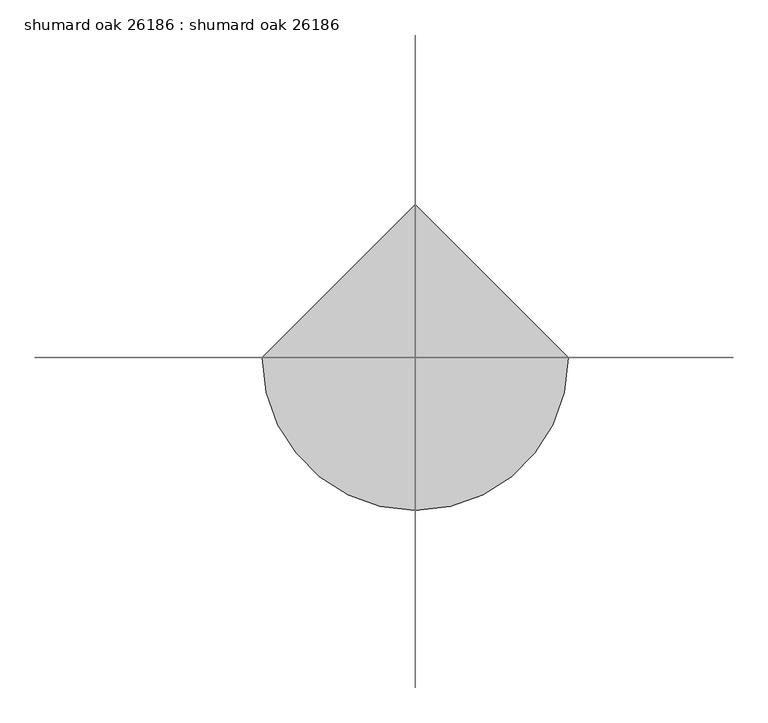
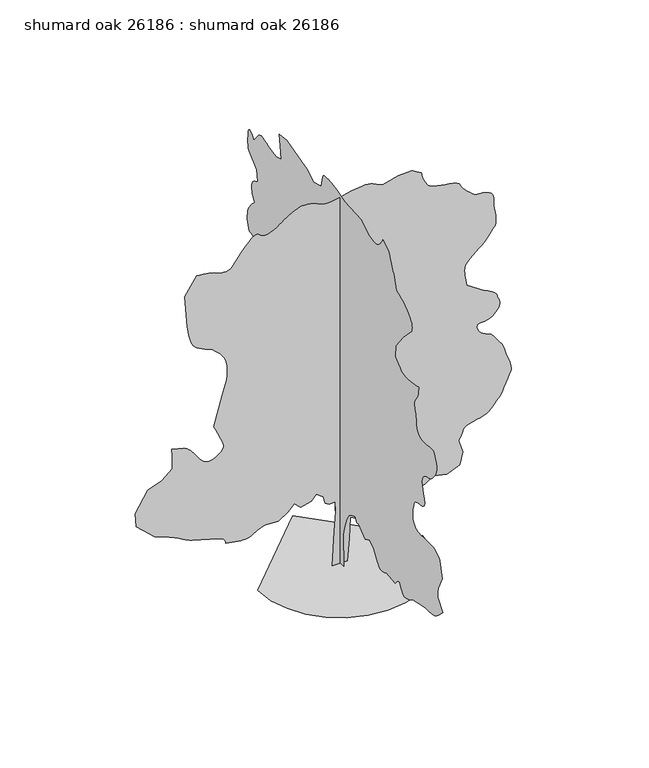
"""IFC4 building model written with IfcOpenShell, lengths in millimetres: proxy geometry, shumard oak 26186 : shumard oak 26186."""

from ifc_helpers import new_model, si_unit, origin, place, context, project, spatial, triangles, source, transform, mapped, element, save


def shumard_oak_26186_shumard_oak_26186_cf07c7db(model_context):
    return source(origin(), model_context, "Body", "Tessellation", [
        triangles([(-0.0016958, 164.6246354, 0.0086022), (-0.0016958, -151.6104316, 0.0086022), (-0.0016958, -124.1113561, 783.7227293), (-0.0016958, -179.1089983, 1017.4612965), (-0.0016958, -261.6049622, 1237.4509209), (-0.0016958, -357.8507226, 1388.6927067), (-0.0016958, -467.8454985, 1457.4403999), (-0.0016958, -605.3383779, 1512.436607), (-0.0016958, -660.3370193, 1388.6927067), (-0.0016958, -756.5828161, 1416.1908829), (-0.0016958, -866.5775557, 1306.195998), (-0.0016958, -1017.8194868, 1209.9502739), (-0.0016958, -1196.5619196, 1292.4469826), (-0.0016958, -1361.5527935, 1182.452243), (-0.0016958, -1471.5476784, 989.9607222), (-0.0016958, -1498.1643677, 951.9597713), (-0.0016958, -1525.3829098, 915.7621988), (-0.0016958, -1553.8031227, 883.1739264), (-0.0016958, -1584.0290394, 855.9959341), (-0.0016958, -1616.658007, 836.0340712), (-0.0016958, -1652.2942039, 825.0891724), (-0.0016958, -1691.5371574, 824.9697756), (-0.0016958, -1729.1774471, 831.662681), (-0.0016958, -1760.3255459, 839.8008471), (-0.0016958, -1786.0582775, 849.1404659), (-0.0016958, -1807.4654011, 859.4426714), (-0.0016958, -1825.6238857, 870.4663445), (-0.0016958, -1841.6182583, 881.9725462), (-0.0016958, -1856.5307201, 893.7149254), (-0.0016958, -2214.0131149, 852.4678791), (-0.0016958, -2249.2480282, 893.1561659), (-0.0016958, -2283.7616192, 930.4738735), (-0.0016958, -2316.8324203, 961.0605967), (-0.0016958, -2347.7391094, 981.54314), (-0.0016958, -2375.7578934, 988.5586275), (-0.0016958, -2400.1697754, 978.7389507), (-0.0016958, -2420.2535786, 948.7136032), (-0.0016958, -2440.416156, 905.5412384), (-0.0016958, -2465.389341, 860.9260838), (-0.0016958, -2494.9323051, 818.4750412), (-0.0016958, -2528.8058189, 781.7974108), (-0.0016958, -2566.7735596, 754.4999491), (-0.0016958, -2608.5820541, 740.1896307), (-0.0016958, -2653.9973053, 742.4730669), (-0.0016958, -2699.5395836, 755.8614212), (-0.0016958, -2742.1861084, 772.1352098), (-0.0016958, -2782.4196991, 790.8169184), (-0.0016958, -2820.7484642, 811.421402), (-0.0016958, -2857.6293526, 833.4686754), (-0.0016958, -2893.5448929, 856.475992), (-0.0016958, -2928.9779045, 879.96591), (-0.0016958, -3423.9482735, 976.2117067), (-0.0016958, -3485.6956673, 976.3335743), (-0.0016958, -3546.579451, 977.174366), (-0.0016958, -3605.7868835, 979.4603456), (-0.0016958, -3662.4543549, 983.9078939), (-0.0016958, -3715.7688332, 991.2459635), (-0.0016958, -3764.8925789, 1002.1882462), (-0.0016958, -3808.9361115, 1017.4612965), (-0.0016958, -3851.3797417, 1039.546649), (-0.0016958, -3896.0075409, 1069.5719965), (-0.0016958, -3942.4134293, 1106.2115479), (-0.0016958, -3990.2924835, 1148.1393665), (-0.0016958, -4039.2383331, 1194.0371464), (-0.0016958, -4088.8951859, 1242.5817123), (-0.0016958, -4138.9334106, 1292.4469826), (-0.0016958, -3946.4265564, 1512.436607), (-0.0016958, -3940.7114983, 1553.6455742), (-0.0016958, -3935.9362083, 1594.6132771), (-0.0016958, -3933.0916145, 1635.0983059), (-0.0016958, -3933.1169037, 1674.8646286), (-0.0016958, -3937.0032944, 1713.6657486), (-0.0016958, -3945.7152626, 1751.2679592), (-0.0016958, -3960.1934486, 1787.4247639), (-0.0016958, -4111.425206, 2103.6601124), (-0.0016958, -4015.1842781, 2488.640538), (-0.0016958, -4007.6405525, 2499.2628548), (-0.0016958, -3985.1869812, 2526.4815422), (-0.0016958, -3948.0776184, 2563.3191193), (-0.0016958, -3896.5156494, 2602.8164177), (-0.0016958, -3830.780127, 2637.9697952), (-0.0016958, -3751.1003975, 2661.820665), (-0.0016958, -3657.7046448, 2667.3831161), (-0.0016958, -3553.6406479, 2663.0650658), (-0.0016958, -3446.4524231, 2661.3634254), (-0.0016958, -3343.1000107, 2661.617189), (-0.0016958, -3250.5928665, 2663.0650658), (-0.0016958, -3175.8660324, 2664.970182), (-0.0016958, -3125.9298363, 2666.6718224), (-0.0016958, -3107.7178665, 2667.3831161), (-0.0016958, -3097.049913, 2674.6474983), (-0.0016958, -3069.5669975, 2695.1200859), (-0.0016958, -3031.9495262, 2726.9207611), (-0.0016958, -2990.9793526, 2768.0688309), (-0.0016958, -2953.3874611, 2816.7097572), (-0.0016958, -2925.9045456, 2870.8625565), (-0.0016958, -2915.2365921, 2928.622403), (-0.0016958, -2917.2431557, 2986.3310898), (-0.0016958, -2922.8564758, 3041.9064766), (-0.0016958, -2931.4672874, 3095.6529053), (-0.0016958, -2942.4907425, 3147.977037), (-0.0016958, -2955.3178665, 3199.2087936), (-0.0016958, -2969.3385223, 3249.7039673), (-0.0016958, -2983.9690247, 3299.8436394), (-0.0016958, -2996.0086967, 3314.52472), (-0.0016958, -3009.4706657, 3328.8250099), (-0.0016958, -3025.8280975, 3342.414006), (-0.0016958, -3046.5038704, 3354.9362068), (-0.0016958, -3072.9705688, 3365.9852417), (-0.0016958, -3106.6510712, 3375.2561874), (-0.0016958, -3148.9673836, 3382.3429642), (-0.0016958, -3200.1485619, 3386.6863037), (-0.0016958, -3255.4443146, 3391.740937), (-0.0016958, -3308.7843727, 3403.2725006), (-0.0016958, -3354.1996239, 3427.0722107), (-0.0016958, -3385.6703773, 3468.9315742), (-0.0016958, -3397.1766518, 3534.5906479), (-0.0016958, -3382.6984657, 3629.8406479), (-0.0016958, -3353.0819595, 3737.5114014), (-0.0016958, -3325.8786781, 3836.2667107), (-0.0016958, -3305.152327, 3925.6746254), (-0.0016958, -3294.9921913, 4005.2023293), (-0.0016958, -3299.5387161, 4074.3920013), (-0.0016958, -3322.8306084, 4132.761113), (-0.0016958, -3368.9571533, 4179.8018463), (-0.0016958, -3425.5228867, 4212.7710548), (-0.0016958, -3477.9993347, 4232.964299), (-0.0016958, -3527.3262657, 4246.1975029), (-0.0016958, -3574.5193153, 4258.2118858), (-0.0016958, -3620.493544, 4274.8233719), (-0.0016958, -3666.2390076, 4301.7473099), (-0.0016958, -3712.6954742, 4344.8004959), (-0.0016958, -3760.0411308, 4399.562851), (-0.0016958, -3805.2023277, 4457.9322533), (-0.0016958, -3844.3694138, 4520.1368866), (-0.0016958, -3873.6809967, 4586.4308052), (-0.0016958, -3889.2765564, 4657.068354), (-0.0016958, -3887.295282, 4732.2777168), (-0.0016958, -3863.9272316, 4812.2879494), (-0.0016958, -3835.7077332, 4887.9545517), (-0.0016958, -3816.632444, 4949.7019455), (-0.0016958, -3799.0047409, 4996.9967331), (-0.0016958, -3775.1032928, 5029.3819656), (-0.0016958, -3737.2573471, 5046.3745331), (-0.0016958, -3677.7705711, 5047.4919067), (-0.0016958, -3588.9466324, 5032.2771378), (-0.0016958, -3483.5620766, 5015.437468), (-0.0016958, -3382.266806, 5012.0591858), (-0.0016958, -3289.150106, 5022.1684525), (-0.0016958, -3208.3018433, 5045.7396881), (-0.0016958, -3143.7860138, 5082.7728928), (-0.0016958, -3099.7421906, 5133.2930649), (-0.0016958, -3080.2096619, 5197.2507889), (-0.0016958, -3073.5295464, 5265.5768509), (-0.0016958, -3065.4015541, 5329.5339935), (-0.0016958, -3056.0541595, 5389.9099594), (-0.0016958, -3045.7417076, 5447.3901718), (-0.0016958, -3034.7182526, 5502.7112137), (-0.0016958, -3023.2119781, 5556.5846695), (-0.0016958, -3011.4772293, 5609.7471222), (-0.0016958, -3000.047113, 5648.0755966), (-0.0016958, -2990.8014565, 5686.505809), (-0.0016958, -2985.8485611, 5725.1900757), (-0.0016958, -2987.423465, 5764.2295532), (-0.0016958, -2997.6341789, 5803.7521408), (-0.0016958, -3018.6907425, 5843.8839935), (-0.0016958, -3052.7267464, 5884.7274307), (-0.0016958, -3089.125106, 5934.8418137), (-0.0016958, -3116.6080215, 5997.6815826), (-0.0016958, -3136.4198936, 6065.8297485), (-0.0016958, -3149.7295464, 6131.8187439), (-0.0016958, -3157.7558006, 6188.1815826), (-0.0016958, -3161.6674805, 6227.450116), (-0.0016958, -3162.7089867, 6242.2073547), (-0.0016958, -3142.4395844, 6237.6861191), (-0.0016958, -3088.0074417, 6226.1798447), (-0.0016958, -3009.0387154, 6210.8383392), (-0.0016958, -2915.160434, 6194.7602509), (-0.0016958, -2815.9731743, 6181.0948059), (-0.0016958, -2721.1295448, 6172.9418152), (-0.0016958, -2640.2304131, 6173.4749222), (-0.0016958, -2571.9299309, 6185.3619873), (-0.0016958, -2507.9599983, 6208.094902), (-0.0016958, -2447.5915901, 6239.8452896), (-0.0016958, -2390.1089069, 6278.808609), (-0.0016958, -2334.7901905, 6323.1826447), (-0.0016958, -2280.9167347, 6371.1634369), (-0.0016958, -2227.7621304, 6420.9476074), (-0.0016958, -2241.5111458, 6709.6945175), (-0.0016958, -2543.9897758, 7094.6826462), (-0.0016958, -2887.7283875, 7452.1625702), (-0.0016958, -2893.1132332, 7496.4860275), (-0.0016958, -2895.3482712, 7541.6722229), (-0.0016958, -2891.335144, 7588.5356415), (-0.0016958, -2877.9493332, 7637.9128601), (-0.0016958, -2852.0666107, 7690.6689423), (-0.0016958, -2810.5377502, 7747.6160477), (-0.0016958, -2750.2379425, 7809.6424942), (-0.0016958, -2679.5242355, 7869.2562973), (-0.0016958, -2608.8108192, 7919.4724182), (-0.0016958, -2538.10467, 7961.8901779), (-0.0016958, -2467.3935791, 7998.0344833), (-0.0016958, -2396.6824883, 8029.5052368), (-0.0016958, -2325.9712521, 8057.8517624), (-0.0016958, -2255.2601612, 8084.6233841), (-0.0016958, -2234.6175259, 8155.1336151), (-0.0016958, -2213.8530956, 8224.4503143), (-0.0016958, -2192.8472557, 8291.3537888), (-0.0016958, -2171.4808273, 8354.651088), (-0.0016958, -2149.6341957, 8413.1219376), (-0.0016958, -2127.1881821, 8465.5983856), (-0.0016958, -2104.0183754, 8510.8607391), (-0.0016958, -2078.3235775, 8560.2129593), (-0.0016958, -2049.9822842, 8621.0970337), (-0.0016958, -2021.4021973, 8686.5529221), (-0.0016958, -1994.9862225, 8749.5955856), (-0.0016958, -1973.1395908, 8803.2917267), (-0.0016958, -1958.2679695, 8840.6039841), (-0.0016958, -1952.7738281, 8854.5996414), (-0.0016958, -1719.0353336, 8992.089505), (-0.0016958, -1707.0516174, 8968.3915329), (-0.0016958, -1693.863905, 8943.9819763), (-0.0016958, -1678.2681999, 8918.1248337), (-0.0016958, -1659.0683544, 8890.1085205), (-0.0016958, -1635.057756, 8859.1970352), (-0.0016958, -1605.0324085, 8824.678212), (-0.0016958, -1567.7934025, 8785.841629), (-0.0016958, -1522.9369835, 8752.2122864), (-0.0016958, -1471.5882282, 8732.2983856), (-0.0016958, -1414.8268673, 8723.7896027), (-0.0016958, -1353.7372822, 8724.4244476), (-0.0016958, -1289.3990582, 8731.9175949), (-0.0016958, -1222.896722, 8743.9825562), (-0.0016958, -1155.3123299, 8758.3334244), (-0.0016958, -852.8259968, 8964.5813004), (-0.0016958, -192.8582863, 9005.8311081), (-0.0016958, -107.5965211, 9029.2756073), (-0.0016958, -23.416737, 9052.008522), (-0.0016958, 58.5983536, 9073.2938507), (-0.0016958, 137.366361, 9092.4200089), (-0.0016958, 211.8051857, 9108.6504135), (-0.0016958, 280.8327856, 9121.2740616), (-0.0016958, 343.3650879, 9129.57995), (-0.0016958, 405.0185557, 9135.9045639), (-0.0016958, 469.5549508, 9141.5181747), (-0.0016958, 533.1311937, 9144.0075577), (-0.0016958, 591.8966838, 9140.9594879), (-0.0016958, 642.0033274, 9129.9863205), (-0.0016958, 679.6029219, 9108.6504135), (-0.0016958, 700.8500261, 9074.5891205), (-0.0016958, 769.5952486, 8799.5832321), (-0.0016958, 1072.081509, 8717.1091965), (-0.0016958, 1347.0698112, 8882.0822662), (-0.0016958, 1690.8031906, 8964.5813004), (-0.0016958, 2144.5313095, 9102.0717453), (-0.0016958, 2447.0174973, 9060.8225189), (-0.0016958, 2419.5169956, 8799.5832321), (-0.0016958, 2364.5209339, 8497.1197174), (-0.0016958, 2584.5030006, 8428.361705), (-0.0016958, 2804.4924797, 8469.6115128), (-0.0016958, 2889.5570549, 8501.5647949), (-0.0016958, 2972.3357231, 8530.7490601), (-0.0016958, 3050.5425774, 8554.3964539), (-0.0016958, 3121.8911293, 8569.7385406), (-0.0016958, 3184.1210518, 8574.0307205), (-0.0016958, 3234.8958595, 8564.480722), (-0.0016958, 3271.9799332, 8538.3439453), (-0.0016958, 3478.2280998, 8290.8712601), (-0.0016958, 3525.090937, 8345.6591949), (-0.0016958, 3570.2521339, 8393.3603531), (-0.0016958, 3612.0606285, 8426.8885391), (-0.0016958, 3648.8144897, 8439.1058167), (-0.0016958, 3678.8373665, 8422.9515701), (-0.0016958, 3700.4526169, 8371.313443), (-0.0016958, 3711.9588913, 8277.1046585), (-0.0016958, 3715.4389114, 8172.4819748), (-0.0016958, 3714.6005905, 8091.684581), (-0.0016958, 3710.155513, 8030.6987686), (-0.0016958, 3702.8149727, 7985.6137299), (-0.0016958, 3693.3152618, 7952.4163376), (-0.0016958, 3682.3679649, 7927.1684601), (-0.0016958, 3670.7093742, 7905.8831314), (-0.0016958, 3354.4789673, 7644.6438446), (-0.0016958, 3326.9707626, 7355.921933), (-0.0016958, 3370.9384277, 7337.989888), (-0.0016958, 3413.6102417, 7318.6346741), (-0.0016958, 3453.615358, 7296.384288), (-0.0016958, 3489.6326363, 7269.8161423), (-0.0016958, 3520.3920959, 7237.4564896), (-0.0016958, 3544.5220184, 7197.8833237), (-0.0016958, 3560.7018448, 7149.674057), (-0.0016958, 3566.8994316, 7096.6389221), (-0.0016958, 3562.9624626, 7043.6032059), (-0.0016958, 3550.618158, 6990.568071), (-0.0016958, 3531.5425781, 6937.5329361), (-0.0016958, 3507.4126556, 6884.4978012), (-0.0016958, 3479.904451, 6831.4626663), (-0.0016958, 3450.7198952, 6778.4269501), (-0.0016958, 3494.7381386, 6734.2313919), (-0.0016958, 3537.6640068, 6689.8829361), (-0.0016958, 3578.4309952, 6645.3060059), (-0.0016958, 3615.9470192, 6600.3732834), (-0.0016958, 3649.1447021, 6554.9580322), (-0.0016958, 3676.9322502, 6508.9329346), (-0.0016958, 3698.2175789, 6462.1968338), (-0.0016958, 3713.4829262, 6416.6548462), (-0.0016958, 3724.4305138, 6374.0080307), (-0.0016958, 3731.7710541, 6333.77444), (-0.0016958, 3736.2161316, 6295.4459656), (-0.0016958, 3738.5020386, 6258.5650772), (-0.0016958, 3739.3400688, 6222.6492462), (-0.0016958, 3739.4670959, 6187.2165253), (-0.0016958, 3656.9680618, 5953.4854431), (-0.0016958, 3618.6901657, 5947.3387253), (-0.0016958, 3580.5140076, 5939.7694199), (-0.0016958, 3542.591613, 5929.304361), (-0.0016958, 3505.0250107, 5914.5215424), (-0.0016958, 3467.9665169, 5893.9477982), (-0.0016958, 3431.4664192, 5866.1599594), (-0.0016958, 3395.728775, 5829.7366013), (-0.0016958, 3363.165937, 5786.4799393), (-0.0016958, 3335.6830215, 5739.6171021), (-0.0016958, 3312.3911293, 5689.7567734), (-0.0016958, 3292.4522301, 5637.4838013), (-0.0016958, 3275.0532921, 5583.4068695), (-0.0016958, 3259.3559944, 5528.1364059), (-0.0016958, 3244.4717285, 5472.2566772), (-0.0016958, 3212.2896812, 5428.0349579), (-0.0016958, 3181.4287743, 5383.7120819), (-0.0016958, 3153.2092758, 5339.1351517), (-0.0016958, 3128.9523262, 5294.1768494), (-0.0016958, 3110.0037735, 5248.7615982), (-0.0016958, 3097.6341797, 5202.7620804), (-0.0016958, 3093.2399712, 5156.026561), (-0.0016958, 3106.9812836, 4784.7797447), (-0.0016958, 3139.1630402, 4781.5284897), (-0.0016958, 3170.049527, 4776.4738564), (-0.0016958, 3198.2690254, 4767.8377556), (-0.0016958, 3222.5006859, 4753.7662308), (-0.0016958, 3241.4745277, 4732.4809021), (-0.0016958, 3253.8188324, 4702.1533928), (-0.0016958, 3258.2383301, 4661.0306122), (-0.0016958, 3257.0192184, 4613.5073502), (-0.0016958, 3253.6665161, 4565.2219254), (-0.0016958, 3248.4848557, 4516.377523), (-0.0016958, 3241.8808983, 4467.0253029), (-0.0016958, 3234.1845657, 4417.3175812), (-0.0016958, 3225.7516502, 4367.3810944), (-0.0016958, 3216.988813, 4317.2922913), (-0.0016958, 3203.2219208, 4042.311692), (-0.0016958, 3464.4612076, 4056.0785843), (-0.0016958, 3753.208699, 4111.0694138), (-0.0016958, 3814.6511696, 4090.2669044), (-0.0016958, 3873.5792587, 4068.37202), (-0.0016958, 3927.4527145, 4044.3182556), (-0.0016958, 3973.7568649, 4017.0132362), (-0.0016958, 4009.9520393, 3985.3901665), (-0.0016958, 4033.523275, 3948.3569618), (-0.0016958, 4041.9306107, 3904.8212471), (-0.0016958, 4039.5429657, 3849.6778107), (-0.0016958, 4032.8119812, 3780.081768), (-0.0016958, 4022.448951, 3698.4716331), (-0.0016958, 4009.2407455, 3607.2347603), (-0.0016958, 3993.8483711, 3508.7840836), (-0.0016958, 3977.00812, 3405.5078293), (-0.0016958, 3959.4568657, 3299.8436394), (-0.0016958, 3835.7077332, 2969.87192), (-0.0016958, 3768.1185448, 2931.9498161), (-0.0016958, 3701.6211502, 2896.3136192), (-0.0016958, 3637.2829262, 2865.2492363), (-0.0016958, 3576.1959572, 2841.0431557), (-0.0016958, 3519.4267479, 2825.9554138), (-0.0016958, 3468.0679642, 2822.3233681), (-0.0016958, 3423.2113998, 2832.3817657), (-0.0016958, 3038.248851, 2997.3548355), (-0.0016958, 2653.2607224, 2873.6312828), (-0.0016958, 2378.2699493, 2681.1244286), (-0.0016958, 2103.2842632, 2268.651059), (-0.0016958, 2076.6675739, 2227.6428062), (-0.0016958, 2049.4488865, 2188.0796688), (-0.0016958, 2021.0263481, 2151.4021111), (-0.0016958, 1990.8027569, 2119.0526321), (-0.0016958, 1958.1739346, 2092.4764927), (-0.0016958, 1922.5377377, 2073.1141571), (-0.0016958, 1883.2946388, 2062.4105953), (-0.0016958, 1844.1303143, 2058.8443886), (-0.0016958, 1807.3715115, 2059.123732), (-0.0016958, 1770.371299, 2062.0498615), (-0.0016958, 1730.4881229, 2066.4186356), (-0.0016958, 1685.070401, 2071.0288193), (-0.0016958, 1631.4762886, 2074.6762711), (-0.0016958, 1567.0592903, 2076.1596107), (-0.0016958, 1497.9510086, 2070.950045), (-0.0016958, 1431.730632, 2056.3577671), (-0.0016958, 1367.9130157, 2033.9498325), (-0.0016958, 1306.020718, 2005.2883553), (-0.0016958, 1245.5712101, 1971.9382107), (-0.0016958, 1186.0844341, 1935.4612221), (-0.0016958, 1127.0801868, 1897.4196487), (-0.0016958, 1044.5834782, 1663.6810089), (-0.0016958, 810.8448383, 1402.4418674), (-0.0016958, 778.5741337, 1367.4862976), (-0.0016958, 741.256426, 1333.2546661), (-0.0016958, 699.7273476, 1299.622562), (-0.0016958, 654.8303061, 1266.4729866), (-0.0016958, 607.408455, 1233.6815289), (-0.0016958, 558.3051295, 1201.1339516), (-0.0016958, 508.3585416, 1168.7032276), (-0.0016958, 425.8618329, 1457.4403999), (-0.0016958, 288.3689717, 1649.9293774), (-0.0016958, 233.3715837, 1526.1856224), (-0.0016958, 192.1232112, 1333.696645), (-0.0016958, 178.3741776, 989.9607222), (-0.0016958, 150.8753565, 508.7344634), (170.3625119, 0.000436, 0.0217742), (-187.1199193, 0.000436, 0.0217742), (-132.1230309, 0.000387, 824.9824928), (-104.6242098, 0.0003581, 1306.2087879), (-118.3734886, 0.0003434, 1553.698914), (-255.8671038, 0.0003442, 1539.9498985), (-352.1128461, 0.000341, 1594.9459602), (-393.359965, 0.0003302, 1773.6885384), (-558.3534187, 0.0003237, 1883.6832779), (-668.3482309, 0.000331, 1759.9395229), (-915.8358135, 0.0003352, 1691.1918297), (-1067.0802881, 0.0003271, 1828.6846001), (-1218.3221466, 0.000336, 1677.4428143), (-1438.311771, 0.0003442, 1539.9498985), (-1768.2961349, 0.0003434, 1553.698914), (-1933.2869362, 0.0003476, 1484.9512207), (-1968.7250347, 0.0003491, 1458.6138748), (-2004.6407204, 0.0003507, 1433.3612011), (-2041.5189926, 0.000352, 1410.2726395), (-2079.8425255, 0.0003531, 1390.4301006), (-2120.0889061, 0.0003541, 1374.915786), (-2162.738047, 0.0003547, 1364.8142223), (-2208.2752384, 0.0003549, 1361.2074657), (-2259.0244663, 0.0003549, 1362.8101295), (-2316.2658852, 0.0003547, 1367.3008438), (-2378.9175842, 0.0003541, 1374.1944637), (-2445.902449, 0.0003536, 1383.0132568), (-2516.1310112, 0.0003531, 1393.2749851), (-2588.5161278, 0.0003523, 1404.4991547), (-2661.9982704, 0.0003518, 1416.2061436), (-2665.4018417, 0.0003499, 1445.5887978), (-2671.5741394, 0.0003481, 1474.4889233), (-2683.2835991, 0.0003465, 1502.428933), (-2703.2986565, 0.0003449, 1528.9262981), (-2734.3630394, 0.0003434, 1553.4981995), (-2779.2448929, 0.0003421, 1575.6648697), (-2840.7382324, 0.000341, 1594.9459602), (-3445.7158401, 0.0003302, 1773.6885384), (-3495.0936401, 0.0003295, 1789.3602562), (-3547.8494316, 0.0003281, 1811.5293972), (-3602.2815742, 0.0003266, 1838.265556), (-3656.7140076, 0.0003247, 1867.6482101), (-3709.469799, 0.0003229, 1897.7523319), (-3758.8728882, 0.0003213, 1926.6550735), (-3803.1957642, 0.0003197, 1952.4285004), (-3850.8716331, 0.0003182, 1977.2011162), (-3910.0790657, 0.0003166, 2004.1403149), (-3978.8876564, 0.0003148, 2032.8804211), (-4055.4181595, 0.0003132, 2063.0657879), (-4137.7140083, 0.0003113, 2094.3332108), (-4223.8456696, 0.0003092, 2126.3194851), (-4311.9327347, 0.0003074, 2158.668964), (-4738.1450912, 0.0002835, 2557.4011665), (-4765.6532959, 0.0002638, 2887.3725952), (-4476.9060951, 0.000236, 3354.8600487), (-4146.9343758, 0.0002287, 3478.6088905), (-3899.4364014, 0.0002163, 3684.8570572), (-3899.4364014, 0.0001977, 4001.0874641), (-3913.2032936, 0.0001877, 4166.0858231), (-3624.4558022, 0.0001919, 4097.3281013), (-3591.9438332, 0.0001932, 4076.3729851), (-3558.8475975, 0.0001945, 4053.3607269), (-3524.5322502, 0.0001961, 4026.2588928), (-3488.4135246, 0.0001979, 3993.03563), (-3449.8815742, 0.0002006, 3951.6082169), (-3408.3524231, 0.0002037, 3899.9953789), (-3363.216806, 0.0002074, 3836.0888145), (-3317.4713425, 0.0002113, 3768.956575), (-3273.4275192, 0.000215, 3709.7491425), (-3229.3839867, 0.0002179, 3659.6856285), (-3183.6385231, 0.0002203, 3619.9601463), (-3134.5403572, 0.0002221, 3591.765937), (-3080.387558, 0.0002229, 3576.3482735), (-3019.4781944, 0.0002229, 3574.8495277), (-2952.9046417, 0.0002221, 3590.0895859), (-2885.848851, 0.0002203, 3620.9507835), (-2822.8567657, 0.0002176, 3662.8860146), (-2768.5513596, 0.0002147, 3711.2984665), (-2727.4541588, 0.0002119, 3761.6413239), (-2704.1622665, 0.000209, 3809.3427727), (-2703.2480782, 0.0002066, 3849.8304176), (-2719.4531937, 0.000204, 3893.6198959), (-2743.5831161, 0.0002006, 3952.5479851), (-2774.3172867, 0.0001961, 4024.0997223), (-2810.3598541, 0.0001914, 4105.735437), (-2850.3649704, 0.0001861, 4194.9657463), (-2893.0114952, 0.0001803, 4289.2506889), (-2936.9788696, 0.0001746, 4386.0755928), (-2744.4975952, 0.0001328, 5087.2685486), (-2718.1576332, 0.0001281, 5166.6433548), (-2692.9100464, 0.0001234, 5244.9263672), (-2669.8216301, 0.0001189, 5321.050209), (-2649.9841782, 0.0001145, 5393.948085), (-2634.4647766, 0.0001105, 5462.477623), (-2624.3555099, 0.0001066, 5525.6220245), (-2620.7487534, 0.0001034, 5582.263916), (-2621.6885216, 0.0001, 5637.5343796), (-2624.7618805, 9.66e-05, 5696.1831253), (-2630.5022278, 9.29e-05, 5756.5079315), (-2639.366803, 8.93e-05, 5816.8333191), (-2651.8128456, 8.58e-05, 5875.4820648), (-2668.3737534, 8.24e-05, 5930.7525284), (-2689.5064751, 7.95e-05, 5980.9936478), (-2716.6844673, 7.67e-05, 6027.7297485), (-2750.3649696, 7.4e-05, 6073.7542648), (-2789.4303177, 7.14e-05, 6119.169516), (-2832.8390053, 6.85e-05, 6164.1022385), (-2879.4986572, 6.59e-05, 6208.6791687), (-2928.3430595, 6.33e-05, 6253.002626), (-2978.2286774, 6.06e-05, 6297.223764), (-3057.4511673, 5.88e-05, 6329.6851547), (-3134.6165154, 5.67e-05, 6362.5273361), (-3207.6922874, 5.49e-05, 6396.0805206), (-3274.6213417, 5.28e-05, 6430.7010818), (-3333.3971146, 5.07e-05, 6466.7942276), (-3381.9365936, 4.83e-05, 6504.6657532), (-3418.2076355, 4.59e-05, 6544.7214478), (-3446.7573463, 4.28e-05, 6598.1123749), (-3473.1478867, 3.86e-05, 6670.5027237), (-3496.8717293, 3.36e-05, 6753.9668152), (-3517.4710533, 2.84e-05, 6840.5557159), (-3534.4636208, 2.34e-05, 6922.3181671), (-3547.3669029, 1.94e-05, 6991.3558136), (-3555.7233696, 1.65e-05, 7039.6918167), (-3610.7144897, -2.94e-05, 7809.6424942), (-3335.7086014, -5.49e-05, 8235.8804306), (-3262.2517479, -5.43e-05, 8226.9396973), (-3189.8616898, -5.38e-05, 8217.4146973), (-3119.6305115, -5.3e-05, 8206.6705856), (-3052.6252991, -5.22e-05, 8194.1225143), (-2989.9887154, -5.15e-05, 8179.162381), (-2932.7372681, -5.04e-05, 8161.2041748), (-2881.9880402, -4.91e-05, 8139.6397934), (-2830.4004913, -4.78e-05, 8118.7864151), (-2772.3107231, -4.7e-05, 8104.2064911), (-2711.3504906, -4.65e-05, 8097.069136), (-2651.1018425, -4.67e-05, 8098.5934616), (-2595.1709541, -4.73e-05, 8109.9724182), (-2547.1901619, -4.86e-05, 8132.4262802), (-2510.7589554, -5.07e-05, 8167.1224182), (-2290.7694763, -6.8e-05, 8455.8699097), (-2232.0038773, -7.19e-05, 8523.1291763), (-2174.2011555, -7.59e-05, 8587.3915329), (-2118.3236069, -7.93e-05, 8645.6333267), (-2065.3290218, -8.22e-05, 8694.8588104), (-2016.1850739, -8.45e-05, 8732.0699112), (-1971.8492626, -8.58e-05, 8754.2185593), (-1933.2869362, -8.61e-05, 8758.3590042), (-1902.260923, -8.53e-05, 8748.0212631), (-1877.0081039, -8.43e-05, 8731.181012), (-1853.1982201, -8.32e-05, 8711.4450073), (-1826.5002857, -8.22e-05, 8692.4455856), (-1792.5886929, -8.11e-05, 8677.7900848), (-1747.1302757, -8.09e-05, 8671.0591003), (-1685.7992809, -8.11e-05, 8675.8593887), (-1612.5227943, -8.24e-05, 8696.712767), (-1537.32346, -8.43e-05, 8731.5112244), (-1465.0070892, -8.69e-05, 8773.9795624), (-1400.3895218, -8.95e-05, 8817.9216476), (-1348.2787491, -9.19e-05, 8857.0378647), (-1313.4833439, -9.35e-05, 8885.1047562), (-1300.8163845, -9.42e-05, 8895.8488678), (-1285.3045406, -9.48e-05, 8905.7802383), (-1244.0574944, -9.63e-05, 8931.6123825), (-1185.0100084, -9.84e-05, 8967.2741592), (-1116.1022959, -0.0001008, 9006.7961655), (-1045.2718082, -0.0001029, 9044.1595825), (-980.4534536, -0.0001047, 9073.344429), (-929.5848289, -0.0001055, 9088.3307236), (-881.3222952, -0.0001058, 9091.6578461), (-821.2740709, -0.0001058, 9089.7021515), (-752.8083372, -0.0001053, 9082.2090042), (-679.2905136, -0.0001045, 9068.9505112), (-604.0912156, -0.0001034, 9049.6714554), (-530.573392, -0.0001019, 9024.1189453), (-462.1076583, -0.0001, 8992.089505), (-389.2730779, -9.84e-05, 8965.9533096), (-302.0062388, -9.79e-05, 8956.4283096), (-202.713753, -9.79e-05, 8960.7204895), (-93.8012603, -9.9e-05, 8976.0625763), (22.3266441, -0.0001003, 8999.7099701), (143.2647473, -0.0001021, 9028.8942352), (266.608781, -0.000104, 9060.8475174), (351.7496415, -0.0001047, 9072.3793716), (435.0871056, -0.0001053, 9082.4886383), (514.8177767, -0.0001058, 9089.7021515), (589.1356968, -0.0001058, 9092.597905), (656.2400311, -0.0001058, 9089.7021515), (714.324785, -0.000105, 9079.5928848), (761.584037, -0.000104, 9060.8475174), (801.2284195, -0.0001026, 9038.8767654), (837.987295, -0.0001016, 9019.8011856), (872.3408667, -0.0001005, 9003.1132507), (904.7690472, -9.98e-05, 8988.356012), (935.7570539, -9.9e-05, 8975.0719391), (965.779858, -9.82e-05, 8962.7017639), (995.3226768, -9.74e-05, 8950.8402786), (1352.8050716, -0.0001032, 9047.0809158), (1669.0404202, -0.000104, 9060.8475174), (1889.0325153, -9.66e-05, 8937.0986755), (1892.1974384, -9.48e-05, 8904.5611267), (1896.6881527, -9.27e-05, 8871.1602585), (1903.8228916, -9.06e-05, 8836.0827484), (1914.9278824, -8.85e-05, 8798.4908569), (1931.3210678, -8.58e-05, 8757.5206833), (1954.3308552, -8.32e-05, 8712.3339066), (1985.2757687, -8.03e-05, 8662.118367), (2016.3831722, -7.74e-05, 8616.1438477), (2042.1971489, -7.56e-05, 8582.1842926), (2067.531213, -7.4e-05, 8557.1398911), (2097.1958267, -7.27e-05, 8537.8358368), (2135.9969467, -7.19e-05, 8521.1990616), (2188.7502674, -7.09e-05, 8504.1047562), (2260.2639256, -6.96e-05, 8483.3781143), (2348.4121788, -6.85e-05, 8463.4136353), (2443.5351517, -6.75e-05, 8448.2500259), (2539.1383278, -6.67e-05, 8434.3055283), (2628.7244293, -6.56e-05, 8417.9478058), (2705.8133286, -6.43e-05, 8395.5701019), (2763.9030968, -6.25e-05, 8363.5918213), (2796.4915146, -5.99e-05, 8318.3794647), (2820.5705681, -5.67e-05, 8265.7507004), (2856.206765, -5.36e-05, 8213.8329391), (2901.4696999, -5.04e-05, 8162.5250244), (2954.4286766, -4.75e-05, 8111.6996384), (3013.1535805, -4.44e-05, 8061.2300446), (3075.7137154, -4.15e-05, 8011.0139236), (3140.2298355, -3.83e-05, 7960.8995407), (3230.9333107, -3.78e-05, 7951.6035965), (3317.928582, -3.73e-05, 7939.5386353), (3397.4559952, -3.62e-05, 7921.9362213), (3465.8073463, -3.47e-05, 7896.027919), (3519.2235626, -3.23e-05, 7859.0708725), (3554.0217293, -2.94e-05, 7808.2966461), (3566.4421921, -2.55e-05, 7740.9100616), (3567.2549332, -2.13e-05, 7670.7044632), (3569.4902618, -1.76e-05, 7612.0812973), (3572.9447021, -1.47e-05, 7563.0337097), (3577.3641998, -1.23e-05, 7521.7077438), (3582.4949913, -1.02e-05, 7486.1732849), (3588.1086021, -8.1e-06, 7454.4484772), (3593.9503967, -6.6e-06, 7424.6799454), (3605.4566711, -2.4e-06, 7354.1947128), (3615.2865944, 1.8e-06, 7285.1832275), (3621.7382355, 5.8e-06, 7219.0413345), (3623.1352432, 9.5e-06, 7157.2177826), (3617.8009758, 1.29e-05, 7101.1851563), (3604.0596634, 1.58e-05, 7052.3666245), (3580.2090843, 1.81e-05, 7012.1836121), (3549.779837, 2.05e-05, 6973.6772415), (3516.9376556, 2.31e-05, 6929.6084198), (3480.9965355, 2.6e-05, 6881.221257), (3441.1948952, 2.89e-05, 6829.7098663), (3396.8208595, 3.2e-05, 6776.2933594), (3347.138427, 3.54e-05, 6722.1408508), (3291.4615929, 3.86e-05, 6668.4452911), (3226.8184456, 4.2e-05, 6613.0986694), (3154.6824417, 4.54e-05, 6553.8912369), (3081.1241409, 4.91e-05, 6492.0421051), (3012.1376541, 5.28e-05, 6428.7453873), (2953.7429626, 5.67e-05, 6365.2196136), (2911.9344681, 6.04e-05, 6302.6338989), (2892.7321518, 6.41e-05, 6242.2329346), (2889.6587929, 6.75e-05, 6182.4918137), (2891.6144875, 7.11e-05, 6121.3286865), (2897.7867851, 7.48e-05, 6058.9464478), (2907.3370743, 7.88e-05, 5995.6241501), (2919.4020355, 8.24e-05, 5931.5652695), (2933.1436386, 8.64e-05, 5867.0238602), (2947.7232719, 9.03e-05, 5802.2533951), (3360.2196053, 0.0001066, 5527.2475067), (3376.1959557, 0.0001071, 5520.1357315), (3417.4457634, 0.0001082, 5500.475885), (3473.8591805, 0.00011, 5470.9864059), (3535.3019417, 0.0001121, 5434.2584152), (3591.7153587, 0.0001147, 5392.9830276), (3632.9648758, 0.0001171, 5349.7525269), (3648.9415169, 0.0001197, 5307.2580276), (3657.5267487, 0.0001221, 5267.1511734), (3677.1610153, 0.0001244, 5227.0193207), (3698.7256874, 0.0001271, 5183.5347656), (3713.0765556, 0.0001302, 5133.2930649), (3711.0699921, 0.0001336, 5072.9682587), (3683.5870766, 0.0001381, 4999.1814835), (3621.4586014, 0.0001436, 4908.5282959), (3535.7588905, 0.0001481, 4831.4141075), (3447.6462456, 0.0001504, 4791.5613075), (3363.1403572, 0.0001515, 4775.7881424), (3288.2612068, 0.0001517, 4770.8096672), (3229.0029053, 0.0001523, 4763.4182579), (3191.4110138, 0.0001536, 4740.4312889), (3181.4796432, 0.0001567, 4688.5388168), (3195.7796425, 0.0001604, 4623.8450912), (3225.2438324, 0.0001635, 4569.9716354), (3267.3316704, 0.0001664, 4525.1153618), (3319.528775, 0.0001685, 4487.4723106), (3379.2948944, 0.0001704, 4455.2396851), (3444.1156471, 0.0001722, 4426.6393959), (3511.4510719, 0.0001738, 4399.8169052), (3578.7612076, 0.0001788, 4314.6761719), (3643.3026169, 0.0001838, 4231.3385262), (3702.3068642, 0.0001885, 4151.6079277), (3753.0055138, 0.000193, 4077.2874641), (3792.6548378, 0.0001972, 4010.1805138), (3818.4611115, 0.0002006, 3952.0907455), (3827.6814789, 0.0002032, 3904.8468269), (3838.9084099, 0.0002066, 3848.3063828), (3866.9753014, 0.0002116, 3767.5086983), (3903.4498192, 0.0002171, 3671.7761696), (3939.9240463, 0.0002231, 3570.531768), (3967.9912285, 0.0002289, 3473.1225975), (3979.2178688, 0.0002342, 3388.9469215), (3965.1716331, 0.0002378, 3327.351844), (3932.583506, 0.0002413, 3266.5442184), (3894.7119804, 0.0002462, 3184.3498169), (3852.9799347, 0.000252, 3089.6076347), (3808.8599533, 0.0002578, 2991.2842758), (3763.7496254, 0.0002633, 2898.2440247), (3719.1471153, 0.000268, 2819.4023254), (3676.4497215, 0.0002714, 2763.6493332), (3635.0475975, 0.0002741, 2719.4784828), (3592.6804161, 0.000277, 2671.193058), (3548.3828293, 0.0002798, 2621.4853363), (3501.189489, 0.0002827, 2572.9967262), (3450.1609177, 0.0002854, 2528.3384056), (3394.3317673, 0.0002877, 2490.1773628), (3332.7114006, 0.0002893, 2461.1552971), (3259.8893921, 0.0002906, 2439.6287041), (3175.9677704, 0.0002919, 2420.2688393), (3088.4646812, 0.000293, 2400.1850361), (3004.822403, 0.0002943, 2376.4944763), (2932.457634, 0.0002961, 2346.3115803), (2878.8638123, 0.0002985, 2306.7459721), (2851.4823441, 0.0003016, 2254.9146881), (2836.8265526, 0.0003048, 2202.96408), (2818.2846611, 0.0003071, 2162.5576801), (2798.8027107, 0.000309, 2130.0888771), (2781.2514565, 0.0003108, 2101.9481529), (2768.5004906, 0.0003124, 2074.5288963), (2763.4461479, 0.0003142, 2044.2240601), (2768.9833099, 0.0003163, 2007.4271782), (2851.4823441, 0.0003321, 1746.1905075), (2782.7499115, 0.0003499, 1443.7041744), (2480.25355, 0.0003573, 1319.9602741), (2177.7672169, 0.0003533, 1388.7054966), (1875.2810291, 0.0003646, 1196.2165192), (1655.2914047, 0.0003573, 1319.9602741), (1339.0560562, 0.0003491, 1457.4531898), (1318.3321758, 0.0003499, 1445.3856125), (1297.0062973, 0.0003507, 1431.6365971), (1274.4790386, 0.0003518, 1414.5220894), (1250.1457855, 0.0003531, 1392.3529484), (1223.4097721, 0.0003547, 1363.4528229), (1193.6663115, 0.000357, 1326.1325718), (1160.3160942, 0.0003599, 1278.7106117), (1125.360597, 0.0003628, 1228.8834206), (1091.1289656, 0.0003654, 1184.8296415), (1057.4968615, 0.0003678, 1145.5866154), (1024.3447426, 0.0003699, 1110.1916828), (991.5558283, 0.0003717, 1077.6822573), (959.0057076, 0.0003736, 1047.0980776), (926.577527, 0.0003754, 1017.4740137), (967.8245733, 0.0003927, 728.7367687), (944.1340136, 0.0003933, 720.0372271), (919.7220589, 0.0003935, 712.1810205), (893.867387, 0.000394, 706.0087955), (865.8460596, 0.0003943, 702.3613438), (834.9418413, 0.0003943, 702.0819277), (800.428323, 0.000394, 706.0087955), (761.584037, 0.0003935, 714.9876806), (721.1370872, 0.0003925, 729.9787714), (682.1353254, 0.0003914, 750.743347), (644.3350164, 0.0003898, 776.3186028), (607.4948233, 0.000388, 805.7419521), (571.3785321, 0.0003862, 838.0508085), (535.7422989, 0.0003841, 872.28244), (500.3473663, 0.000382, 907.4792015), (239.1089334, 0.0003738, 1044.9720446), (211.6111206, 0.000404, 536.2452115), (-1916.7566952, 0.0, 0.0), (-1866.0836254, -439.194304, 0.0), (-1721.7683064, -842.5237186, 0.0), (-1495.3652653, -1198.4313549, 0.0), (-1198.4313549, -1495.3652653, 0.0), (-842.5237186, -1721.7683064, 0.0), (-439.194304, -1866.0836254, 0.0), (8.38e-05, -1916.7566952, 0.0), (439.194304, -1866.0836254, 0.0), (842.5237186, -1721.7683064, 0.0), (1198.4313549, -1495.3652653, 0.0), (1495.3652653, -1198.4313549, 0.0), (1721.7683064, -842.5237186, 0.0), (1866.0836254, -439.194304, 0.0), (1916.7566952, 0.0001675, 0.0), (-0.0002514, 1916.7566952, 0.0)], [[407, 408, 409], [173, 174, 175], [406, 407, 409], [219, 220, 221], [1, 2, 3], [414, 1, 3], [413, 414, 3], [413, 3, 4], [412, 413, 4], [412, 4, 5], [255, 256, 257], [219, 221, 222], [65, 66, 67], [405, 406, 409], [8, 9, 10], [219, 222, 223], [404, 405, 409], [64, 65, 67], [412, 5, 6], [411, 412, 6], [403, 404, 409], [219, 223, 224], [172, 173, 175], [172, 175, 176], [171, 172, 176], [171, 176, 177], [170, 171, 177], [254, 255, 257], [254, 257, 258], [402, 403, 409], [63, 64, 67], [218, 219, 224], [401, 402, 409], [218, 224, 225], [217, 218, 225], [312, 313, 314], [216, 217, 225], [216, 225, 226], [170, 177, 178], [169, 170, 178], [168, 169, 178], [167, 168, 178], [167, 178, 179], [166, 167, 179], [166, 179, 180], [165, 166, 180], [11, 12, 13], [216, 226, 227], [215, 216, 227], [400, 401, 409], [400, 409, 410], [399, 400, 410], [29, 30, 31], [62, 63, 67], [214, 215, 227], [214, 227, 228], [410, 411, 6], [410, 6, 7], [165, 180, 181], [164, 165, 181], [312, 314, 315], [61, 62, 67], [213, 214, 228], [60, 61, 67], [59, 60, 67], [58, 59, 67], [57, 58, 67], [56, 57, 67], [55, 56, 67], [54, 55, 67], [53, 54, 67], [52, 53, 67], [52, 67, 68], [52, 68, 69], [253, 254, 258], [252, 253, 258], [29, 31, 32], [271, 272, 273], [271, 273, 274], [270, 271, 274], [270, 274, 275], [269, 270, 275], [268, 269, 275], [268, 275, 276], [268, 276, 277], [268, 277, 278], [268, 278, 279], [268, 279, 280], [268, 280, 281], [268, 281, 282], [268, 282, 283], [267, 268, 283], [266, 267, 283], [265, 266, 283], [264, 265, 283], [263, 264, 283], [262, 263, 283], [261, 262, 283], [260, 261, 283], [259, 260, 283], [259, 283, 284], [52, 69, 70], [212, 213, 228], [212, 228, 229], [211, 212, 229], [210, 211, 229], [209, 210, 229], [208, 209, 229], [10, 11, 13], [163, 164, 181], [163, 181, 182], [312, 315, 316], [51, 52, 70], [51, 70, 71], [51, 71, 72], [207, 208, 229], [207, 229, 230], [206, 207, 230], [366, 367, 368], [74, 75, 76], [74, 76, 77], [74, 77, 78], [74, 78, 79], [74, 79, 80], [74, 80, 81], [74, 81, 82], [74, 82, 83], [74, 83, 84], [74, 84, 85], [74, 85, 86], [73, 74, 86], [73, 86, 87], [73, 87, 88], [72, 73, 88], [51, 72, 88], [51, 88, 89], [51, 89, 90], [51, 90, 91], [51, 91, 92], [51, 92, 93], [50, 51, 93], [49, 50, 93], [48, 49, 93], [47, 48, 93], [46, 47, 93], [45, 46, 93], [44, 45, 93], [43, 44, 93], [42, 43, 93], [41, 42, 93], [40, 41, 93], [39, 40, 93], [38, 39, 93], [37, 38, 93], [36, 37, 93], [35, 36, 93], [35, 93, 94], [34, 35, 94], [34, 94, 95], [34, 95, 96], [33, 34, 96], [205, 206, 230], [258, 259, 284], [252, 258, 284], [29, 32, 33], [29, 33, 96], [29, 96, 97], [311, 312, 316], [190, 191, 192], [190, 192, 193], [190, 193, 194], [190, 194, 195], [190, 195, 196], [190, 196, 197], [190, 197, 198], [190, 198, 199], [190, 199, 200], [190, 200, 201], [190, 201, 202], [190, 202, 203], [190, 203, 204], [190, 204, 205], [189, 190, 205], [189, 205, 230], [189, 230, 231], [189, 231, 232], [189, 232, 233], [189, 233, 234], [410, 7, 8], [310, 311, 316], [310, 316, 317], [309, 310, 317], [308, 309, 317], [307, 308, 317], [306, 307, 317], [305, 306, 317], [304, 305, 317], [303, 304, 317], [302, 303, 317], [302, 317, 318], [301, 302, 318], [300, 301, 318], [299, 300, 318], [299, 318, 319], [298, 299, 319], [298, 319, 320], [162, 163, 182], [366, 368, 369], [298, 320, 321], [366, 369, 370], [366, 370, 371], [366, 371, 372], [366, 372, 373], [366, 373, 374], [366, 374, 375], [365, 366, 375], [364, 365, 375], [363, 364, 375], [362, 363, 375], [361, 362, 375], [360, 361, 375], [359, 360, 375], [358, 359, 375], [357, 358, 375], [356, 357, 375], [355, 356, 375], [354, 355, 375], [353, 354, 375], [352, 353, 375], [351, 352, 375], [350, 351, 375], [350, 375, 376], [234, 235, 236], [189, 234, 236], [188, 189, 236], [188, 236, 237], [188, 237, 238], [188, 238, 239], [188, 239, 240], [188, 240, 241], [188, 241, 242], [188, 242, 243], [188, 243, 244], [188, 244, 245], [188, 245, 246], [188, 246, 247], [188, 247, 248], [188, 248, 249], [188, 249, 250], [188, 250, 251], [188, 251, 252], [188, 252, 284], [187, 188, 284], [187, 284, 285], [187, 285, 286], [187, 286, 287], [187, 287, 288], [187, 288, 289], [187, 289, 290], [187, 290, 291], [187, 291, 292], [187, 292, 293], [187, 293, 294], [187, 294, 295], [187, 295, 296], [187, 296, 297], [187, 297, 298], [187, 298, 321], [187, 321, 322], [187, 322, 323], [187, 323, 324], [187, 324, 325], [187, 325, 326], [187, 326, 327], [187, 327, 328], [187, 328, 329], [187, 329, 330], [187, 330, 331], [187, 331, 332], [187, 332, 333], [187, 333, 334], [187, 334, 335], [186, 187, 335], [185, 186, 335], [184, 185, 335], [183, 184, 335], [182, 183, 335], [162, 182, 335], [161, 162, 335], [160, 161, 335], [159, 160, 335], [158, 159, 335], [157, 158, 335], [156, 157, 335], [155, 156, 335], [154, 155, 335], [153, 154, 335], [152, 153, 335], [151, 152, 335], [150, 151, 335], [350, 376, 377], [142, 143, 144], [142, 144, 145], [141, 142, 145], [141, 145, 146], [140, 141, 146], [140, 146, 147], [139, 140, 147], [138, 139, 147], [137, 138, 147], [136, 137, 147], [135, 136, 147], [134, 135, 147], [133, 134, 147], [133, 147, 148], [132, 133, 148], [131, 132, 148], [130, 131, 148], [129, 130, 148], [128, 129, 148], [127, 128, 148], [127, 148, 149], [126, 127, 149], [125, 126, 149], [125, 149, 150], [125, 150, 335], [124, 125, 335], [123, 124, 335], [122, 123, 335], [121, 122, 335], [120, 121, 335], [119, 120, 335], [118, 119, 335], [117, 118, 335], [116, 117, 335], [115, 116, 335], [114, 115, 335], [113, 114, 335], [112, 113, 335], [111, 112, 335], [110, 111, 335], [109, 110, 335], [108, 109, 335], [107, 108, 335], [106, 107, 335], [105, 106, 335], [104, 105, 335], [103, 104, 335], [102, 103, 335], [101, 102, 335], [100, 101, 335], [99, 100, 335], [98, 99, 335], [97, 98, 335], [29, 97, 335], [28, 29, 335], [27, 28, 335], [26, 27, 335], [25, 26, 335], [25, 335, 336], [25, 336, 337], [25, 337, 338], [349, 350, 377], [339, 340, 341], [338, 339, 341], [338, 341, 342], [338, 342, 343], [338, 343, 344], [338, 344, 345], [338, 345, 346], [348, 349, 377], [347, 348, 377], [346, 347, 377], [338, 346, 377], [20, 21, 22], [19, 20, 22], [19, 22, 23], [18, 19, 23], [17, 18, 23], [17, 23, 24], [17, 24, 25], [16, 17, 25], [15, 16, 25], [14, 15, 25], [14, 25, 338], [13, 14, 338], [10, 13, 338], [8, 10, 338], [8, 338, 377], [410, 8, 377], [398, 399, 410], [398, 410, 377], [397, 398, 377], [396, 397, 377], [395, 396, 377], [394, 395, 377], [393, 394, 377], [393, 377, 378], [392, 393, 378], [391, 392, 378], [390, 391, 378], [389, 390, 378], [389, 378, 379], [389, 379, 380], [388, 389, 380], [388, 380, 381], [387, 388, 381], [387, 381, 382], [386, 387, 382], [386, 382, 383], [385, 386, 383], [384, 385, 383], [472, 473, 474], [415, 416, 417], [793, 415, 417], [792, 793, 417], [792, 417, 418], [776, 777, 778], [776, 778, 779], [776, 779, 780], [776, 780, 781], [776, 781, 782], [776, 782, 783], [776, 783, 784], [776, 784, 785], [776, 785, 786], [776, 786, 787], [776, 787, 788], [776, 788, 789], [443, 444, 445], [471, 472, 474], [471, 474, 475], [471, 475, 476], [471, 476, 477], [471, 477, 478], [471, 478, 479], [471, 479, 480], [471, 480, 481], [471, 481, 482], [776, 789, 790], [776, 790, 791], [539, 540, 541], [759, 760, 761], [471, 482, 483], [424, 425, 426], [423, 424, 426], [539, 541, 542], [613, 614, 615], [756, 757, 758], [756, 758, 759], [755, 756, 759], [539, 542, 543], [538, 539, 543], [538, 543, 544], [538, 544, 545], [538, 545, 546], [538, 546, 547], [538, 547, 548], [538, 548, 549], [538, 549, 550], [754, 755, 759], [471, 483, 484], [538, 550, 551], [537, 538, 551], [443, 445, 446], [792, 418, 419], [536, 537, 551], [535, 536, 551], [534, 535, 551], [533, 534, 551], [532, 533, 551], [531, 532, 551], [530, 531, 551], [529, 530, 551], [528, 529, 551], [527, 528, 551], [526, 527, 551], [525, 526, 551], [524, 525, 551], [524, 551, 552], [523, 524, 552], [522, 523, 552], [522, 552, 553], [521, 522, 553], [520, 521, 553], [519, 520, 553], [613, 615, 616], [420, 421, 422], [419, 420, 422], [612, 613, 616], [612, 616, 617], [612, 617, 618], [612, 618, 619], [776, 791, 792], [776, 792, 419], [775, 776, 419], [774, 775, 419], [773, 774, 419], [772, 773, 419], [771, 772, 419], [770, 771, 419], [769, 770, 419], [768, 769, 419], [767, 768, 419], [766, 767, 419], [765, 766, 419], [764, 765, 419], [466, 467, 468], [466, 468, 469], [466, 469, 470], [465, 466, 470], [464, 465, 470], [463, 464, 470], [462, 463, 470], [461, 462, 470], [461, 470, 471], [461, 471, 484], [461, 484, 485], [461, 485, 486], [460, 461, 486], [459, 460, 486], [459, 486, 487], [458, 459, 487], [457, 458, 487], [456, 457, 487], [455, 456, 487], [454, 455, 487], [453, 454, 487], [452, 453, 487], [451, 452, 487], [451, 487, 488], [451, 488, 489], [450, 451, 489], [450, 489, 490], [449, 450, 490], [449, 490, 491], [449, 491, 492], [448, 449, 492], [518, 519, 553], [518, 553, 554], [611, 612, 619], [611, 619, 620], [611, 620, 621], [448, 492, 493], [754, 759, 761], [754, 761, 762], [753, 754, 762], [752, 753, 762], [501, 502, 503], [611, 621, 622], [763, 764, 419], [447, 448, 493], [517, 518, 554], [500, 501, 503], [611, 622, 623], [762, 763, 419], [762, 419, 422], [752, 762, 422], [751, 752, 422], [750, 751, 422], [749, 750, 422], [748, 749, 422], [747, 748, 422], [747, 422, 423], [427, 428, 429], [517, 554, 555], [426, 427, 429], [517, 555, 556], [516, 517, 556], [516, 556, 557], [516, 557, 558], [516, 558, 559], [516, 559, 560], [516, 560, 561], [516, 561, 562], [516, 562, 563], [516, 563, 564], [516, 564, 565], [516, 565, 566], [516, 566, 567], [516, 567, 568], [516, 568, 569], [516, 569, 570], [516, 570, 571], [515, 516, 571], [515, 571, 572], [514, 515, 572], [514, 572, 573], [442, 443, 446], [442, 446, 447], [442, 447, 493], [441, 442, 493], [440, 441, 493], [439, 440, 493], [438, 439, 493], [437, 438, 493], [436, 437, 493], [435, 436, 493], [434, 435, 493], [433, 434, 493], [432, 433, 493], [431, 432, 493], [430, 431, 493], [429, 430, 493], [426, 429, 493], [426, 493, 494], [423, 426, 494], [423, 494, 495], [747, 423, 495], [747, 495, 496], [746, 747, 496], [746, 496, 497], [746, 497, 498], [746, 498, 499], [746, 499, 500], [746, 500, 503], [746, 503, 504], [746, 504, 505], [746, 505, 506], [746, 506, 507], [746, 507, 508], [746, 508, 509], [746, 509, 510], [746, 510, 511], [746, 511, 512], [745, 746, 512], [745, 512, 513], [745, 513, 514], [745, 514, 573], [745, 573, 574], [745, 574, 575], [745, 575, 576], [745, 576, 577], [745, 577, 578], [745, 578, 579], [745, 579, 580], [745, 580, 581], [745, 581, 582], [745, 582, 583], [745, 583, 584], [745, 584, 585], [745, 585, 586], [745, 586, 587], [745, 587, 588], [745, 588, 589], [745, 589, 590], [745, 590, 591], [745, 591, 592], [745, 592, 593], [745, 593, 594], [745, 594, 595], [745, 595, 596], [745, 596, 597], [745, 597, 598], [745, 598, 599], [745, 599, 600], [745, 600, 601], [745, 601, 602], [745, 602, 603], [745, 603, 604], [745, 604, 605], [745, 605, 606], [745, 606, 607], [745, 607, 608], [745, 608, 609], [745, 609, 610], [745, 610, 611], [745, 611, 623], [745, 623, 624], [745, 624, 625], [745, 625, 626], [745, 626, 627], [745, 627, 628], [745, 628, 629], [745, 629, 630], [745, 630, 631], [745, 631, 632], [745, 632, 633], [745, 633, 634], [745, 634, 635], [745, 635, 636], [712, 713, 714], [647, 648, 649], [646, 647, 649], [645, 646, 649], [645, 649, 650], [644, 645, 650], [644, 650, 651], [643, 644, 651], [643, 651, 652], [642, 643, 652], [642, 652, 653], [642, 653, 654], [642, 654, 655], [642, 655, 656], [642, 656, 657], [642, 657, 658], [642, 658, 659], [642, 659, 660], [642, 660, 661], [642, 661, 662], [642, 662, 663], [642, 663, 664], [642, 664, 665], [642, 665, 666], [642, 666, 667], [642, 667, 668], [642, 668, 669], [642, 669, 670], [642, 670, 671], [642, 671, 672], [641, 642, 672], [641, 672, 673], [640, 641, 673], [640, 673, 674], [639, 640, 674], [639, 674, 675], [638, 639, 675], [637, 638, 675], [637, 675, 676], [636, 637, 676], [690, 691, 692], [690, 692, 693], [689, 690, 693], [688, 689, 693], [725, 726, 727], [725, 727, 728], [724, 725, 728], [724, 728, 729], [723, 724, 729], [723, 729, 730], [722, 723, 730], [722, 730, 731], [721, 722, 731], [721, 731, 732], [721, 732, 733], [721, 733, 734], [721, 734, 735], [721, 735, 736], [721, 736, 737], [721, 737, 738], [721, 738, 739], [721, 739, 740], [721, 740, 741], [721, 741, 742], [721, 742, 743], [721, 743, 744], [721, 744, 745], [720, 721, 745], [719, 720, 745], [718, 719, 745], [717, 718, 745], [716, 717, 745], [715, 716, 745], [714, 715, 745], [712, 714, 745], [711, 712, 745], [710, 711, 745], [709, 710, 745], [708, 709, 745], [707, 708, 745], [687, 688, 693], [636, 676, 677], [687, 693, 694], [686, 687, 694], [685, 686, 694], [685, 694, 695], [685, 695, 696], [685, 696, 697], [685, 697, 698], [685, 698, 699], [685, 699, 700], [685, 700, 701], [685, 701, 702], [685, 702, 703], [685, 703, 704], [684, 685, 704], [684, 704, 705], [684, 705, 706], [706, 707, 745], [684, 706, 745], [683, 684, 745], [682, 683, 745], [681, 682, 745], [680, 681, 745], [636, 677, 678], [745, 636, 678], [745, 678, 679], [680, 745, 679], [808, 809, 794], [807, 808, 794], [807, 794, 795], [806, 807, 795], [806, 795, 796], [806, 796, 797], [805, 806, 797], [804, 805, 797], [804, 797, 798], [804, 798, 799], [804, 799, 800], [804, 800, 801], [804, 801, 802], [804, 802, 803]], closed=False),
    ])


if __name__ == "__main__":
    model = new_model("IFC4")
    model_context = context("Model", 3, world=origin())
    ifc_project = project(units=[si_unit("LENGTHUNIT", "METRE", prefix="MILLI")], contexts=[model_context])
    site = spatial("IfcSite", under=ifc_project)
    building = spatial("IfcBuilding", under=site)
    placement = place(None, origin())
    shumard_oak_26186_shumard_oak_26186_shape = shumard_oak_26186_shumard_oak_26186_cf07c7db(model_context)
    element("IfcBuildingElementProxy", 1, Name="shumard oak 26186 : shumard oak 26186", ObjectType="shumard oak 26186 : shumard oak 26186", at=placement, inside=building, context=model_context, shape_type="MappedRepresentation", body=[
        mapped(shumard_oak_26186_shumard_oak_26186_shape, transform((0.0, 0.0, 0.0), x_axis=(1.0, 0.0, 0.0), y_axis=(0.0, 1.0, 0.0), z_axis=(0.0, 0.0, 1.0))),
    ])
    save(model, "model.ifc")

# Revit data of these elements
# Type "shumard oak 26186 : shumard oak 26186"
#   built-in parameter 1005195 = "RPC-16-FXGQ-AS80-PNHH-0000-ST1L-LVER-AU"
#   Height = 0
